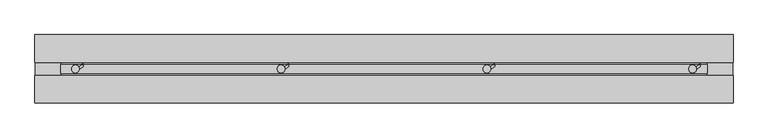
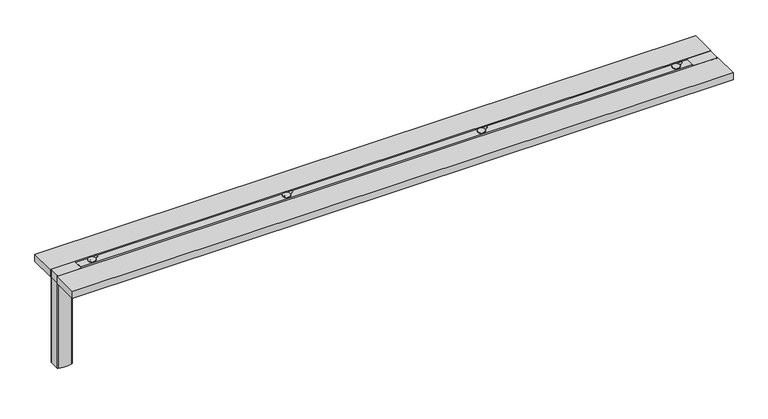
"""IFC4 building model written with IfcOpenShell, lengths in millimetres: proxy geometry, Bandalux_Draperies_Estrada-HorizontalTrackBase_2 : Draperies - Estrada Track - FOSCA FR Sand."""

from ifc_helpers import new_model, si_unit, point, frame, frame_2d, origin, place, context, project, spatial, polyline, circle_curve, trimmed, segment, composite_curve, outline, extrude, source, transform, mapped, element, save
from ifc_brep_helpers import plane_surface, cylinder_surface, advanced_brep


def generic_models_0eca5815(model_context):
    return source(origin(), model_context, "Body", "SolidModel", [
        advanced_brep(
        [(-354.4483333, 0.0, 2629.7), (-354.4753523, -0.8657872, 2629.7), (-382.2183333, 0.0, 2629.7), (-356.8294844, 7.7752611, 2629.7), (-354.4483333, 0.0, 2631.49), (-356.8294844, 7.7752611, 2631.49), (-382.2183333, 0.0, 2631.49), (-354.4753523, -0.8657872, 2631.49)],
        [
            (0, 1, circle_curve(frame((-368.3333333, 0.0, 2629.7), z_axis=(0.0, 0.0, -1.0), x_axis=(-1.0, 0.0, 0.0)), 13.885)),
            (1, 2, circle_curve(frame((-368.3333333, 0.0, 2629.7), z_axis=(0.0, 0.0, -1.0), x_axis=(-1.0, 0.0, 0.0)), 13.885)),
            (2, 3, circle_curve(frame((-368.3333333, 0.0, 2629.7), z_axis=(0.0, 0.0, -1.0), x_axis=(-1.0, 0.0, 0.0)), 13.885)),
            (3, 0, circle_curve(frame((-368.3333333, 0.0, 2629.7), z_axis=(0.0, 0.0, -1.0), x_axis=(-1.0, 0.0, 0.0)), 13.885)),
            (4, 5, circle_curve(frame((-368.3333333, 0.0, 2631.49), z_axis=(0.0, 0.0, 1.0), x_axis=(-1.0, 0.0, 0.0)), 13.885)),
            (5, 6, circle_curve(frame((-368.3333333, 0.0, 2631.49), z_axis=(0.0, 0.0, 1.0), x_axis=(-1.0, 0.0, 0.0)), 13.885)),
            (6, 7, circle_curve(frame((-368.3333333, 0.0, 2631.49), z_axis=(0.0, 0.0, 1.0), x_axis=(-1.0, 0.0, 0.0)), 13.885)),
            (7, 4, circle_curve(frame((-368.3333333, 0.0, 2631.49), z_axis=(0.0, 0.0, 1.0), x_axis=(-1.0, 0.0, 0.0)), 13.885)),
            (0, 4),
            (6, 2),
        ],
        [
            plane_surface(frame((-382.2183333, 0.0, 2629.7), z_axis=(0.0, 0.0, -1.0), x_axis=(0.0, 1.0, 0.0))),
            plane_surface(frame((-382.2183333, 0.0, 2631.49), z_axis=(0.0, 0.0, 1.0), x_axis=(0.0, -1.0, 0.0))),
            cylinder_surface(frame((-368.3333333, 0.0, 2631.49), z_axis=(0.0, 0.0, -1.0), x_axis=(-1.0, 0.0, 0.0)), 13.885),
        ],
        [
            (0, [[1, 2, 3, 4]]),
            (1, [[5, 6, 7, 8]]),
            (2, [[9, -8, -7, 10, -2, -1]]),
            (2, [[-9, -4, -3, -10, -6, -5]]),
        ],
    ),
        extrude(outline(composite_curve([segment(polyline([(18.1222089, 2628.2777911), (18.1222089, 2624.7025827), (16.7, 2624.7025827), (16.7, 2629.7)]), True, "CONTINUOUS"), segment(trimmed(circle_curve(frame_2d((16.7, 2628.2777911)), 1.4222089), [point((16.7, 2629.7))], [point((18.1222089, 2628.2777911))], False, "CARTESIAN"), True, "CONTINUOUS")], self_intersect=False)), frame((-344.3333333, 0.0, 0.0), z_axis=(1.0, 0.0, 0.0), x_axis=(0.0, 1.0, 0.0)), (0.0, 0.0, 1.0), 3.991695),
        extrude(outline(composite_curve([segment(polyline([(-362.562708, 3.521006), (-344.3333333, 16.7), (-340.3416383, 16.7), (-340.3416383, 9.2460587), (-362.9887858, -6.76), (-368.3333333, -6.76)]), True, "CONTINUOUS"), segment(trimmed(circle_curve(frame_2d((-368.3333333, 0.0)), 6.76), [point((-368.3333333, -6.76))], [point((-375.0933333, 0.0))], False, "CARTESIAN"), True, "CONTINUOUS"), segment(trimmed(circle_curve(frame_2d((-368.3333333, 0.0)), 6.76), [point((-375.0933333, 0.0))], [point((-362.562708, 3.521006))], False, "CARTESIAN"), True, "CONTINUOUS")], self_intersect=False)), frame((0.0, 0.0, 2628.3), z_axis=(0.0, 0.0, 1.0), x_axis=(1.0, 0.0, 0.0)), (0.0, 0.0, 1.0), 1.4),
        advanced_brep(
        [(382.2183333, 0.0, 2629.7), (382.1913143, -0.8657872, 2629.7), (354.4483333, 0.0, 2629.7), (379.8371823, 7.7752611, 2629.7), (382.2183333, 0.0, 2631.49), (379.8371823, 7.7752611, 2631.49), (354.4483333, 0.0, 2631.49), (382.1913143, -0.8657872, 2631.49)],
        [
            (0, 1, circle_curve(frame((368.3333333, 0.0, 2629.7), z_axis=(0.0, 0.0, -1.0), x_axis=(-1.0, 0.0, 0.0)), 13.885)),
            (1, 2, circle_curve(frame((368.3333333, 0.0, 2629.7), z_axis=(0.0, 0.0, -1.0), x_axis=(-1.0, 0.0, 0.0)), 13.885)),
            (2, 3, circle_curve(frame((368.3333333, 0.0, 2629.7), z_axis=(0.0, 0.0, -1.0), x_axis=(-1.0, 0.0, 0.0)), 13.885)),
            (3, 0, circle_curve(frame((368.3333333, 0.0, 2629.7), z_axis=(0.0, 0.0, -1.0), x_axis=(-1.0, 0.0, 0.0)), 13.885)),
            (4, 5, circle_curve(frame((368.3333333, 0.0, 2631.49), z_axis=(0.0, 0.0, 1.0), x_axis=(-1.0, 0.0, 0.0)), 13.885)),
            (5, 6, circle_curve(frame((368.3333333, 0.0, 2631.49), z_axis=(0.0, 0.0, 1.0), x_axis=(-1.0, 0.0, 0.0)), 13.885)),
            (6, 7, circle_curve(frame((368.3333333, 0.0, 2631.49), z_axis=(0.0, 0.0, 1.0), x_axis=(-1.0, 0.0, 0.0)), 13.885)),
            (7, 4, circle_curve(frame((368.3333333, 0.0, 2631.49), z_axis=(0.0, 0.0, 1.0), x_axis=(-1.0, 0.0, 0.0)), 13.885)),
            (0, 4),
            (6, 2),
        ],
        [
            plane_surface(frame((354.4483333, 0.0, 2629.7), z_axis=(0.0, 0.0, -1.0), x_axis=(0.0, 1.0, 0.0))),
            plane_surface(frame((354.4483333, 0.0, 2631.49), z_axis=(0.0, 0.0, 1.0), x_axis=(0.0, -1.0, 0.0))),
            cylinder_surface(frame((368.3333333, 0.0, 2631.49), z_axis=(0.0, 0.0, -1.0), x_axis=(-1.0, 0.0, 0.0)), 13.885),
        ],
        [
            (0, [[1, 2, 3, 4]]),
            (1, [[5, 6, 7, 8]]),
            (2, [[9, -8, -7, 10, -2, -1]]),
            (2, [[-9, -4, -3, -10, -6, -5]]),
        ],
    ),
        extrude(outline(composite_curve([segment(polyline([(18.1222089, 2628.2777911), (18.1222089, 2624.7025827), (16.7, 2624.7025827), (16.7, 2629.7)]), True, "CONTINUOUS"), segment(trimmed(circle_curve(frame_2d((16.7, 2628.2777911)), 1.4222089), [point((16.7, 2629.7))], [point((18.1222089, 2628.2777911))], False, "CARTESIAN"), True, "CONTINUOUS")], self_intersect=False)), frame((392.3333333, 0.0, 0.0), z_axis=(1.0, 0.0, 0.0), x_axis=(0.0, 1.0, 0.0)), (0.0, 0.0, 1.0), 3.991695),
        extrude(outline(composite_curve([segment(polyline([(374.1039587, 3.521006), (392.3333333, 16.7), (396.3250283, 16.7), (396.3250283, 9.2460587), (373.6778809, -6.76), (368.3333333, -6.76)]), True, "CONTINUOUS"), segment(trimmed(circle_curve(frame_2d((368.3333333, 0.0)), 6.76), [point((368.3333333, -6.76))], [point((361.5733333, 0.0))], False, "CARTESIAN"), True, "CONTINUOUS"), segment(trimmed(circle_curve(frame_2d((368.3333333, 0.0)), 6.76), [point((361.5733333, 0.0))], [point((374.1039587, 3.521006))], False, "CARTESIAN"), True, "CONTINUOUS")], self_intersect=False)), frame((0.0, 0.0, 2628.3), z_axis=(0.0, 0.0, 1.0), x_axis=(1.0, 0.0, 0.0)), (0.0, 0.0, 1.0), 1.4),
        advanced_brep(
        [(-1091.115, 0.0, 2629.7), (-1091.142019, -0.8657872, 2629.7), (-1118.885, 0.0, 2629.7), (-1093.4961511, 7.7752611, 2629.7), (-1091.115, 0.0, 2631.49), (-1093.4961511, 7.7752611, 2631.49), (-1118.885, 0.0, 2631.49), (-1091.142019, -0.8657872, 2631.49)],
        [
            (0, 1, circle_curve(frame((-1105.0, 0.0, 2629.7), z_axis=(0.0, 0.0, -1.0), x_axis=(-1.0, 0.0, 0.0)), 13.885)),
            (1, 2, circle_curve(frame((-1105.0, 0.0, 2629.7), z_axis=(0.0, 0.0, -1.0), x_axis=(-1.0, 0.0, 0.0)), 13.885)),
            (2, 3, circle_curve(frame((-1105.0, 0.0, 2629.7), z_axis=(0.0, 0.0, -1.0), x_axis=(-1.0, 0.0, 0.0)), 13.885)),
            (3, 0, circle_curve(frame((-1105.0, 0.0, 2629.7), z_axis=(0.0, 0.0, -1.0), x_axis=(-1.0, 0.0, 0.0)), 13.885)),
            (4, 5, circle_curve(frame((-1105.0, 0.0, 2631.49), z_axis=(0.0, 0.0, 1.0), x_axis=(-1.0, 0.0, 0.0)), 13.885)),
            (5, 6, circle_curve(frame((-1105.0, 0.0, 2631.49), z_axis=(0.0, 0.0, 1.0), x_axis=(-1.0, 0.0, 0.0)), 13.885)),
            (6, 7, circle_curve(frame((-1105.0, 0.0, 2631.49), z_axis=(0.0, 0.0, 1.0), x_axis=(-1.0, 0.0, 0.0)), 13.885)),
            (7, 4, circle_curve(frame((-1105.0, 0.0, 2631.49), z_axis=(0.0, 0.0, 1.0), x_axis=(-1.0, 0.0, 0.0)), 13.885)),
            (0, 4),
            (6, 2),
        ],
        [
            plane_surface(frame((-1118.885, 0.0, 2629.7), z_axis=(0.0, 0.0, -1.0), x_axis=(0.0, 1.0, 0.0))),
            plane_surface(frame((-1118.885, 0.0, 2631.49), z_axis=(0.0, 0.0, 1.0), x_axis=(0.0, -1.0, 0.0))),
            cylinder_surface(frame((-1105.0, 0.0, 2631.49), z_axis=(0.0, 0.0, -1.0), x_axis=(-1.0, 0.0, 0.0)), 13.885),
        ],
        [
            (0, [[1, 2, 3, 4]]),
            (1, [[5, 6, 7, 8]]),
            (2, [[9, -8, -7, 10, -2, -1]]),
            (2, [[-9, -4, -3, -10, -6, -5]]),
        ],
    ),
        extrude(outline(composite_curve([segment(polyline([(18.1222089, 2628.2777911), (18.1222089, 2624.7025827), (16.7, 2624.7025827), (16.7, 2629.7)]), True, "CONTINUOUS"), segment(trimmed(circle_curve(frame_2d((16.7, 2628.2777911)), 1.4222089), [point((16.7, 2629.7))], [point((18.1222089, 2628.2777911))], False, "CARTESIAN"), True, "CONTINUOUS")], self_intersect=False)), frame((-1081.0, 0.0, 0.0), z_axis=(1.0, 0.0, 0.0), x_axis=(0.0, 1.0, 0.0)), (0.0, 0.0, 1.0), 3.991695),
        extrude(outline(composite_curve([segment(polyline([(-1099.2293746, 3.521006), (-1081.0, 16.7), (-1077.008305, 16.7), (-1077.008305, 9.2460587), (-1099.6554524, -6.76), (-1105.0, -6.76)]), True, "CONTINUOUS"), segment(trimmed(circle_curve(frame_2d((-1105.0, 0.0)), 6.76), [point((-1105.0, -6.76))], [point((-1111.76, 0.0))], False, "CARTESIAN"), True, "CONTINUOUS"), segment(trimmed(circle_curve(frame_2d((-1105.0, 0.0)), 6.76), [point((-1111.76, 0.0))], [point((-1099.2293746, 3.521006))], False, "CARTESIAN"), True, "CONTINUOUS")], self_intersect=False)), frame((0.0, 0.0, 2628.3), z_axis=(0.0, 0.0, 1.0), x_axis=(1.0, 0.0, 0.0)), (0.0, 0.0, 1.0), 1.4),
        advanced_brep(
        [(1118.885, 0.0, 2629.7), (1118.857981, -0.8657872, 2629.7), (1091.115, 0.0, 2629.7), (1116.5038489, 7.7752611, 2629.7), (1118.885, 0.0, 2631.49), (1116.5038489, 7.7752611, 2631.49), (1091.115, 0.0, 2631.49), (1118.857981, -0.8657872, 2631.49)],
        [
            (0, 1, circle_curve(frame((1105.0, 0.0, 2629.7), z_axis=(0.0, 0.0, -1.0), x_axis=(-1.0, 0.0, 0.0)), 13.885)),
            (1, 2, circle_curve(frame((1105.0, 0.0, 2629.7), z_axis=(0.0, 0.0, -1.0), x_axis=(-1.0, 0.0, 0.0)), 13.885)),
            (2, 3, circle_curve(frame((1105.0, 0.0, 2629.7), z_axis=(0.0, 0.0, -1.0), x_axis=(-1.0, 0.0, 0.0)), 13.885)),
            (3, 0, circle_curve(frame((1105.0, 0.0, 2629.7), z_axis=(0.0, 0.0, -1.0), x_axis=(-1.0, 0.0, 0.0)), 13.885)),
            (4, 5, circle_curve(frame((1105.0, 0.0, 2631.49), z_axis=(0.0, 0.0, 1.0), x_axis=(-1.0, 0.0, 0.0)), 13.885)),
            (5, 6, circle_curve(frame((1105.0, 0.0, 2631.49), z_axis=(0.0, 0.0, 1.0), x_axis=(-1.0, 0.0, 0.0)), 13.885)),
            (6, 7, circle_curve(frame((1105.0, 0.0, 2631.49), z_axis=(0.0, 0.0, 1.0), x_axis=(-1.0, 0.0, 0.0)), 13.885)),
            (7, 4, circle_curve(frame((1105.0, 0.0, 2631.49), z_axis=(0.0, 0.0, 1.0), x_axis=(-1.0, 0.0, 0.0)), 13.885)),
            (0, 4),
            (6, 2),
        ],
        [
            plane_surface(frame((1091.115, 0.0, 2629.7), z_axis=(0.0, 0.0, -1.0), x_axis=(0.0, 1.0, 0.0))),
            plane_surface(frame((1091.115, 0.0, 2631.49), z_axis=(0.0, 0.0, 1.0), x_axis=(0.0, -1.0, 0.0))),
            cylinder_surface(frame((1105.0, 0.0, 2631.49), z_axis=(0.0, 0.0, -1.0), x_axis=(-1.0, 0.0, 0.0)), 13.885),
        ],
        [
            (0, [[1, 2, 3, 4]]),
            (1, [[5, 6, 7, 8]]),
            (2, [[9, -8, -7, 10, -2, -1]]),
            (2, [[-9, -4, -3, -10, -6, -5]]),
        ],
    ),
        extrude(outline(composite_curve([segment(polyline([(18.1222089, 2628.2777911), (18.1222089, 2624.7025827), (16.7, 2624.7025827), (16.7, 2629.7)]), True, "CONTINUOUS"), segment(trimmed(circle_curve(frame_2d((16.7, 2628.2777911)), 1.4222089), [point((16.7, 2629.7))], [point((18.1222089, 2628.2777911))], False, "CARTESIAN"), True, "CONTINUOUS")], self_intersect=False)), frame((1129.0, 0.0, 0.0), z_axis=(1.0, 0.0, 0.0), x_axis=(0.0, 1.0, 0.0)), (0.0, 0.0, 1.0), 3.991695),
        extrude(outline(composite_curve([segment(polyline([(1110.7706254, 3.521006), (1129.0, 16.7), (1132.991695, 16.7), (1132.991695, 9.2460587), (1110.3445476, -6.76), (1105.0, -6.76)]), True, "CONTINUOUS"), segment(trimmed(circle_curve(frame_2d((1105.0, 0.0)), 6.76), [point((1105.0, -6.76))], [point((1098.24, 0.0))], False, "CARTESIAN"), True, "CONTINUOUS"), segment(trimmed(circle_curve(frame_2d((1105.0, 0.0)), 6.76), [point((1098.24, 0.0))], [point((1110.7706254, 3.521006))], False, "CARTESIAN"), True, "CONTINUOUS")], self_intersect=False)), frame((0.0, 0.0, 2628.3), z_axis=(0.0, 0.0, 1.0), x_axis=(1.0, 0.0, 0.0)), (0.0, 0.0, 1.0), 1.4),
        extrude(outline(polyline([(-1250.0, 122.75), (1250.0, 122.75), (1250.0, 22.75), (-1250.0, 22.75), (-1250.0, 122.75)])), frame((0.0, 0.0, 2600.0), z_axis=(0.0, 0.0, 1.0), x_axis=(1.0, 0.0, 0.0)), (0.0, 0.0, 1.0), 28.3),
        extrude(outline(polyline([(-1250.0, -22.75), (1250.0, -22.75), (1250.0, -122.75), (-1250.0, -122.75), (-1250.0, -22.75)])), frame((0.0, 0.0, 2600.0), z_axis=(0.0, 0.0, 1.0), x_axis=(1.0, 0.0, 0.0)), (0.0, 0.0, 1.0), 28.3),
        extrude(outline(polyline([(-1157.5, 16.0), (1157.5, 16.0), (1157.5, -16.0), (-1157.5, -16.0), (-1157.5, 16.0)])), frame((0.0, 0.0, 2600.0), z_axis=(0.0, 0.0, 1.0), x_axis=(1.0, 0.0, 0.0)), (0.0, 0.0, 1.0), 28.3),
        extrude(outline(composite_curve([segment(trimmed(circle_curve(frame_2d((-1219.8, 74.7)), 100.2), [point((-1194.1814172, -22.1696455))], [point((-1245.4185828, -22.1696455))], False, "CARTESIAN"), True, "CONTINUOUS"), segment(trimmed(circle_curve(frame_2d((-1244.1402104, -17.3358308)), 5.0), [point((-1245.4185828, -22.1696455))], [point((-1249.115673, -17.8305749))], False, "CARTESIAN"), True, "CONTINUOUS"), segment(trimmed(circle_curve(frame_2d((-1069.8, 0.0)), 180.2), [point((-1249.115673, -17.8305749))], [point((-1249.115673, 17.8305749))], False, "CARTESIAN"), True, "CONTINUOUS"), segment(trimmed(circle_curve(frame_2d((-1244.1402104, 17.3358308)), 5.0), [point((-1249.115673, 17.8305749))], [point((-1245.4185828, 22.1696455))], False, "CARTESIAN"), True, "CONTINUOUS"), segment(trimmed(circle_curve(frame_2d((-1219.8, -74.7)), 100.2), [point((-1245.4185828, 22.1696455))], [point((-1194.1814172, 22.1696455))], False, "CARTESIAN"), True, "CONTINUOUS"), segment(trimmed(circle_curve(frame_2d((-1195.4597896, 17.3358308)), 5.0), [point((-1194.1814172, 22.1696455))], [point((-1190.4843269, 17.8305749))], False, "CARTESIAN"), True, "CONTINUOUS"), segment(trimmed(circle_curve(frame_2d((-1369.8, 0.0)), 180.2), [point((-1190.4843269, 17.8305749))], [point((-1190.4843269, -17.8305749))], False, "CARTESIAN"), True, "CONTINUOUS"), segment(trimmed(circle_curve(frame_2d((-1195.4597896, -17.3358308)), 5.0), [point((-1190.4843269, -17.8305749))], [point((-1194.1814172, -22.1696455))], False, "CARTESIAN"), True, "CONTINUOUS")], self_intersect=False)), frame((0.0, 0.0, 2258.3), z_axis=(0.0, 0.0, 1.0), x_axis=(1.0, 0.0, 0.0)), (0.0, 0.0, 1.0), 340.0),
        extrude(outline(composite_curve([segment(trimmed(circle_curve(frame_2d((-1162.5, 18.0)), 5.0), [point((-1162.5, 23.0))], [point((-1157.5, 18.0))], False, "CARTESIAN"), True, "CONTINUOUS"), segment(polyline([(-1157.5, 18.0), (-1157.5, -18.0)]), True, "CONTINUOUS"), segment(trimmed(circle_curve(frame_2d((-1162.5, -18.0)), 5.0), [point((-1157.5, -18.0))], [point((-1162.5, -23.0))], False, "CARTESIAN"), True, "CONTINUOUS"), segment(polyline([(-1162.5, -23.0), (-1197.5570236, -23.0)]), True, "CONTINUOUS"), segment(trimmed(circle_curve(frame_2d((-1219.8, 74.7)), 100.2), [point((-1197.5570236, -23.0))], [point((-1245.4185828, -22.1696455))], False, "CARTESIAN"), True, "CONTINUOUS"), segment(trimmed(circle_curve(frame_2d((-1244.1402104, -17.3358308)), 5.0), [point((-1245.4185828, -22.1696455))], [point((-1249.115673, -17.8305749))], False, "CARTESIAN"), True, "CONTINUOUS"), segment(trimmed(circle_curve(frame_2d((-1069.8, 0.0)), 180.2), [point((-1249.115673, -17.8305749))], [point((-1249.115673, 17.8305749))], False, "CARTESIAN"), True, "CONTINUOUS"), segment(trimmed(circle_curve(frame_2d((-1244.1402104, 17.3358308)), 5.0), [point((-1249.115673, 17.8305749))], [point((-1245.4185828, 22.1696455))], False, "CARTESIAN"), True, "CONTINUOUS"), segment(trimmed(circle_curve(frame_2d((-1219.8, -74.7)), 100.2), [point((-1245.4185828, 22.1696455))], [point((-1197.5570236, 23.0))], False, "CARTESIAN"), True, "CONTINUOUS"), segment(polyline([(-1197.5570236, 23.0), (-1162.5, 23.0)]), True, "CONTINUOUS")], self_intersect=False)), frame((0.0, 0.0, 2598.3), z_axis=(0.0, 0.0, 1.0), x_axis=(1.0, 0.0, 0.0)), (0.0, 0.0, 1.0), 30.0),
        extrude(outline(composite_curve([segment(polyline([(1162.5, 23.0), (1197.5570236, 23.0)]), True, "CONTINUOUS"), segment(trimmed(circle_curve(frame_2d((1219.8, -74.7)), 100.2), [point((1197.5570236, 23.0))], [point((1245.4185828, 22.1696455))], False, "CARTESIAN"), True, "CONTINUOUS"), segment(trimmed(circle_curve(frame_2d((1244.1402104, 17.3358308)), 5.0), [point((1245.4185828, 22.1696455))], [point((1249.115673, 17.8305749))], False, "CARTESIAN"), True, "CONTINUOUS"), segment(trimmed(circle_curve(frame_2d((1069.8, 0.0)), 180.2), [point((1249.115673, 17.8305749))], [point((1249.115673, -17.8305749))], False, "CARTESIAN"), True, "CONTINUOUS"), segment(trimmed(circle_curve(frame_2d((1244.1402104, -17.3358308)), 5.0), [point((1249.115673, -17.8305749))], [point((1245.4185828, -22.1696455))], False, "CARTESIAN"), True, "CONTINUOUS"), segment(trimmed(circle_curve(frame_2d((1219.8, 74.7)), 100.2), [point((1245.4185828, -22.1696455))], [point((1197.5570236, -23.0))], False, "CARTESIAN"), True, "CONTINUOUS"), segment(polyline([(1197.5570236, -23.0), (1162.5, -23.0)]), True, "CONTINUOUS"), segment(trimmed(circle_curve(frame_2d((1162.5, -18.0)), 5.0), [point((1162.5, -23.0))], [point((1157.5, -18.0))], False, "CARTESIAN"), True, "CONTINUOUS"), segment(polyline([(1157.5, -18.0), (1157.5, 18.0)]), True, "CONTINUOUS"), segment(trimmed(circle_curve(frame_2d((1162.5, 18.0)), 5.0), [point((1157.5, 18.0))], [point((1162.5, 23.0))], False, "CARTESIAN"), True, "CONTINUOUS")], self_intersect=False)), frame((0.0, 0.0, 2598.3), z_axis=(0.0, 0.0, 1.0), x_axis=(1.0, 0.0, 0.0)), (0.0, 0.0, 1.0), 30.0),
    ])


if __name__ == "__main__":
    model = new_model("IFC4")
    model_context = context("Model", 3, world=origin())
    ifc_project = project(units=[si_unit("LENGTHUNIT", "METRE", prefix="MILLI")], contexts=[model_context])
    site = spatial("IfcSite", under=ifc_project)
    building = spatial("IfcBuilding", under=site)
    placement = place(None, origin())
    generic_models_shape = generic_models_0eca5815(model_context)
    element("IfcBuildingElementProxy", 1, Name="Bandalux_Draperies_Estrada-HorizontalTrackBase_2 : Draperies - Estrada Track - FOSCA FR Sand", ObjectType="Bandalux_Draperies_Estrada-HorizontalTrackBase_2 : Draperies - Estrada Track - FOSCA FR Sand", at=placement, inside=building, context=model_context, shape_type="MappedRepresentation", body=[
        mapped(generic_models_shape, transform((0.0, 0.0, 0.0), x_axis=(1.0, 0.0, 0.0), y_axis=(0.0, 1.0, 0.0), z_axis=(0.0, 0.0, 1.0))),
    ])
    save(model, "model.ifc")

# Revit data of these elements
# Project information
#   Project Issue Date = "Issue Date"
#   Project Status = "Project Status"
#   Client Name = "Owner"
#   Project Address = "Enter address here"
#   Project Name = "Project Name"
#   Project Number = "0001"
# Type "Bandalux_Draperies_Estrada-HorizontalTrackBase_2 : Draperies - Estrada Track - FOSCA FR Sand"
#   · Type of Operating System · [instance default] = "Motor (Cable)"
#   · Side of Operating System · [instance default] = "Right Side"
#   · Mounting Option · [instance default] = "Ceiling Bracket"
#   · Draperies Stacking · [instance default] = "RLA"
#   · Draperies Length · [instance default] = "Floor"
#   · Fabric Options · [instance default] = "Single Fabric"
#   Warning [instance default] = "No Warnings"
#   URL = "https://bandalux.com/"
#   Revit Version = "Revit 2020 - English"
#   Review Date = "08/23"
#   Product URL = "https://contract.bandalux.com/en/draperies"
#   Model = "Draperies - Estrada Track - Horizontal Track / Horizontal Base"
#   Manufacturer = "Bandalux"
#   IfcExportAs = "IfcShadingDevice.SHUTTER"
#   Family Version = "1.0"
#   Export Type to IFC As = "IfcShadingDevice.SHUTTER"
#   Description = "Bandalux’s traditional shades boast fire-resistant and thermal and acoustic insulation properties. This makes them ideal for public buildings such as hotels, schools, projection halls, gyms, and other places that have to comply with building regulations.\n\nThey are elegant and highly decorative solutions that can be combined with other systems, including the roller shade and the sliding panel. The Estrada track offers a silent and powerful motor drive option for draperies. The motor can be operated in three ways: by pulling the draperies fabric, by remote control or by wall-mounted push button.\n\nThe motor can be installed on both sides of the track and the fabric is manufactured in such a way that it hides the view of the motor (max. surface area 24 m2). The track can be curved for spaces with curved walls or as a room divider.\n\nFor outdoor installation, they are also available with the Polyscreen® fabric for pergolas and porches."
#   Created by = "BIMETRICAL"
#   BIMETRICAL = "http://www.bimetrical.com/"
#   HP_Shd-Wdth-Cntrl [instance default] = 1500 mm
#   HP_Shd-Hght-Cntrl [instance default] = 2000 mm
#   HP_Mxml-Shd-Wdth [instance default] = 6000 mm
#   HP_Mxml-Shd-Hght [instance default] = 5000 mm
#   HP_Mnml-Shd-Wdth [instance default] = 400 mm
#   HP_Mnml-Shd-Hght [instance default] = 400 mm
#   Width [instance default] = 1500 mm
#   Height [instance default] = 2000 mm
#   · Number of Brackets · [instance default] = 3
#   WRNG [instance default] = 0
#   Right/Left Side [instance default] = yes
#   RLO [instance default] = no
#   RLA [instance default] = yes
#   RAL [instance default] = no
#   Puddle [instance default] = no
#   Motor Symbology [instance default] = no
#   Motor (Cable) [instance default] = yes
#   HP_Vi2 [instance default] = no
#   HP_Vi1 [instance default] = yes
#   Floor [instance default] = yes
#   Draperies Stacking [instance default] = no
#   Single/Double Fabric [instance default] = no
#   Clearance Area [instance default] = yes
#   Ceiling Bracket [instance default] = yes
#   CSOS [instance default] = 2
#   COP [instance default] = 2
#   CO [instance default] = 2
#   CFS [instance default] = 2
#   CM = 4
#   Break [instance default] = no
#   Default Elevation = 0
# Element 1 (IfcBuildingElementProxy, "Bandalux_Draperies_Estrada-HorizontalTrackBase_2 : Draperies - Estrada Track - FOSCA FR Sand")
#   HP_Shd-Wdth-Cntrl = 2500 mm
#   HP_Shd-Hght-Cntrl = 2600 mm
#   Width = 2500 mm
#   Height = 2600 mm
#   · Number of Brackets · = 4
#   Materials on its faces: "White RAL 9010", "Generic_Clearance Area"
# Materials
#   "White RAL 9010": class "Paint/Coating Bandalux", colour RGB 241 236 225, transparency 0, Manufacturer = "Bandalux", URL = "https://bandalux.com", Description = "White RAL 9010", Cost = 0
#   "Generic_Clearance Area": class "Generic Bandalux", colour RGB 229 229 229, transparency 0.8, URL = "https://bandalux.com", Cost = 0
